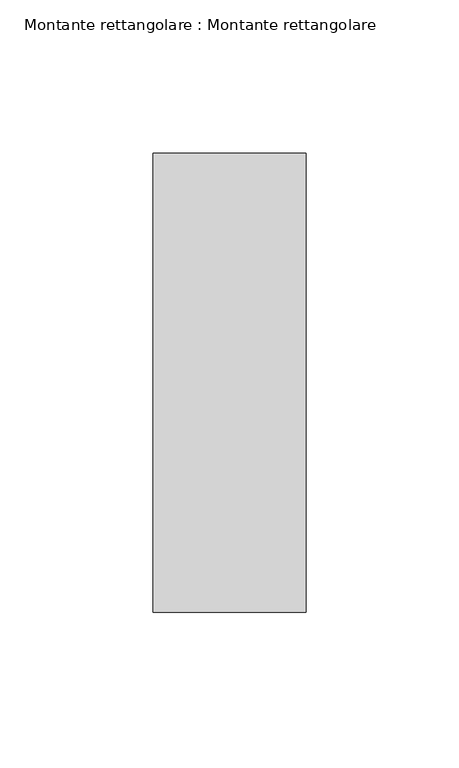
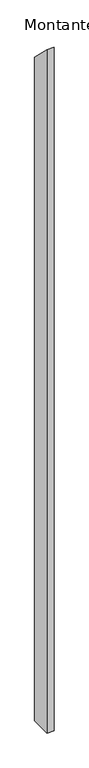
"""IFC4 building model written with IfcOpenShell, lengths in millimetres: member geometry, Montante rettangolare : Montante rettangolare."""

from ifc_helpers import new_model, si_unit, frame, origin, place, context, project, spatial, polyline, outline, extrude, source, transform, mapped, element, save


def montante_rettangolare_montante_rettangolare_df59e700(model_context):
    return source(origin(), model_context, "Body", "SweptSolid", [
        extrude(outline(polyline([(-75.0, 75.0), (75.0, -75.0), (75.0, -5005.0), (-75.0, -5005.0), (-75.0, 75.0)])), frame((-50.0, 0.0, 0.0), z_axis=(1.0, 0.0, 0.0), x_axis=(0.0, 1.0, 0.0)), (0.0, 0.0, 1.0), 50.0),
    ])


if __name__ == "__main__":
    model = new_model("IFC4")
    model_context = context("Model", 3, world=origin())
    ifc_project = project(units=[si_unit("LENGTHUNIT", "METRE", prefix="MILLI")], contexts=[model_context])
    site = spatial("IfcSite", under=ifc_project)
    building = spatial("IfcBuilding", under=site)
    placement = place(None, origin())
    montante_rettangolare_montante_rettangolare_shape = montante_rettangolare_montante_rettangolare_df59e700(model_context)
    element("IfcMember", 1, ObjectType="Montante rettangolare : Montante rettangolare", at=placement, inside=building, context=model_context, shape_type="MappedRepresentation", body=[
        mapped(montante_rettangolare_montante_rettangolare_shape, transform((0.0, 0.0, 0.0), x_axis=(1.0, 0.0, 0.0), y_axis=(0.0, 1.0, 0.0), z_axis=(0.0, 0.0, 1.0))),
    ])
    save(model, "model.ifc")

# Revit data of these elements
# Type "Montante rettangolare : Montante rettangolare"
#   built-in parameter 1007304 = 0.492126 (stored number, unit not read)
#   built-in parameter 1007301 = 0.082021 (stored number, unit not read)
#   built-in parameter 1007300 = 0.082021 (stored number, unit not read)
# Element 1 (IfcMember, "Montante rettangolare : Montante rettangolare")
#   Materials on its faces: "Acciaio"
# Materials
#   "Acciaio": class "Metallo", colour RGB 247 247 247, transparency 0, Description = "Acciaio, finitura zigrinata", Cost = 0
